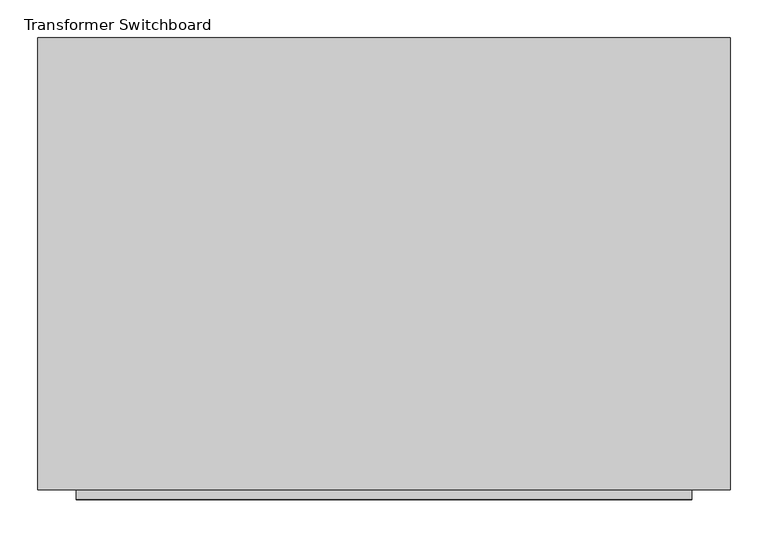
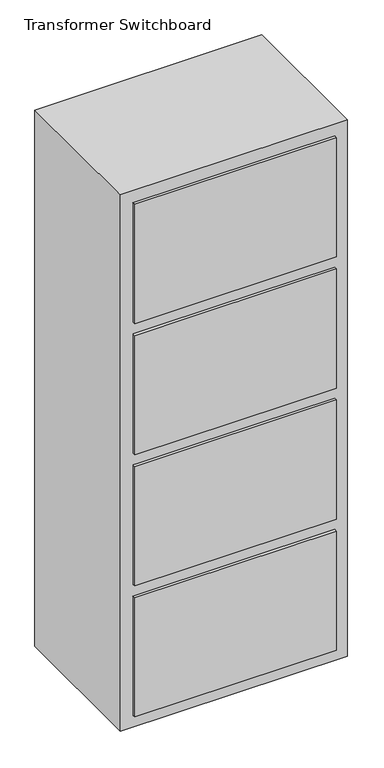
"""IFC4 building model written with IfcOpenShell, lengths in millimetres: proxy geometry, Transformer Switchboard."""

from ifc_helpers import new_model, si_unit, frame, origin, origin_with_axes, place, context, project, spatial, polyline, outline, extrude, source, transform, mapped, element, save


def transformer_switchboard_ad6aeb5d(model_context):
    return source(origin(), model_context, "Body", "SweptSolid", [
        extrude(outline(polyline([(406.4, -609.6), (-406.4, -609.6), (-406.4, -596.9), (406.4, -596.9), (406.4, -609.6)])), frame((0.0, 0.0, 1727.2), z_axis=(0.0, 0.0, 1.0), x_axis=(1.0, 0.0, 0.0)), (0.0, 0.0, 1.0), 508.0),
        extrude(outline(polyline([(406.4, -609.6), (-406.4, -609.6), (-406.4, -596.9), (406.4, -596.9), (406.4, -609.6)])), frame((0.0, 0.0, 1168.4), z_axis=(0.0, 0.0, 1.0), x_axis=(1.0, 0.0, 0.0)), (0.0, 0.0, 1.0), 508.0),
        extrude(outline(polyline([(406.4, -609.6), (-406.4, -609.6), (-406.4, -596.9), (406.4, -596.9), (406.4, -609.6)])), frame((0.0, 0.0, 609.6), z_axis=(0.0, 0.0, 1.0), x_axis=(1.0, 0.0, 0.0)), (0.0, 0.0, 1.0), 508.0),
        extrude(outline(polyline([(406.4, -609.6), (-406.4, -609.6), (-406.4, -596.9), (406.4, -596.9), (406.4, -609.6)])), frame((0.0, 0.0, 50.8), z_axis=(0.0, 0.0, 1.0), x_axis=(1.0, 0.0, 0.0)), (0.0, 0.0, 1.0), 508.0),
        extrude(outline(polyline([(457.2, 0.0), (457.2, -596.9), (-457.2, -596.9), (-457.2, 0.0), (457.2, 0.0)])), origin_with_axes(), (0.0, 0.0, 1.0), 2286.0),
    ])


if __name__ == "__main__":
    model = new_model("IFC4")
    model_context = context("Model", 3, world=origin())
    ifc_project = project(units=[si_unit("LENGTHUNIT", "METRE", prefix="MILLI")], contexts=[model_context])
    site = spatial("IfcSite", under=ifc_project)
    building = spatial("IfcBuilding", under=site)
    placement = place(None, origin())
    transformer_switchboard_shape = transformer_switchboard_ad6aeb5d(model_context)
    element("IfcBuildingElementProxy", 1, Name="Transformer Switchboard : 24\"deep x 36\" wide x 90\"H", ObjectType="Transformer Switchboard : 24\"deep x 36\" wide x 90\"H", at=placement, inside=building, context=model_context, shape_type="MappedRepresentation", body=[
        mapped(transformer_switchboard_shape, transform((0.0, 0.0, 0.0), x_axis=(1.0, 0.0, 0.0), y_axis=(0.0, 1.0, 0.0), z_axis=(0.0, 0.0, 1.0))),
    ])
    save(model, "model.ifc")

# Revit data of these elements
# Type "Transformer Switchboard : 24\"deep x 36\" wide x 90\"H"
#   Type Mark = "SG-1"
#   Switchboard Width = 2' - 0"
#   Switchboard Length = 3' - 0"
#   Switchboard Height = 7' - 6"
#   Primary Voltage = 480 V
#   Panel Length = 2' - 8"
#   Panel Height = 1' - 8"
#   Length 1 = 3' - 0"
#   Height 1 = 7' - 6"
#   Half Switchboard Length = 1' - 6"
#   Clearance_Side_Back = 2' - 0"
#   Clearance_Front = 5' - 0"
#   Primary Number of Poles = 3
#   Switchboard Material = none
#   Load Classification = Other
